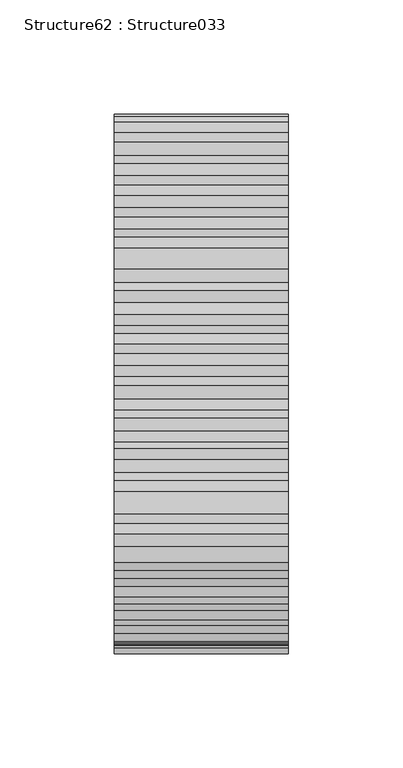
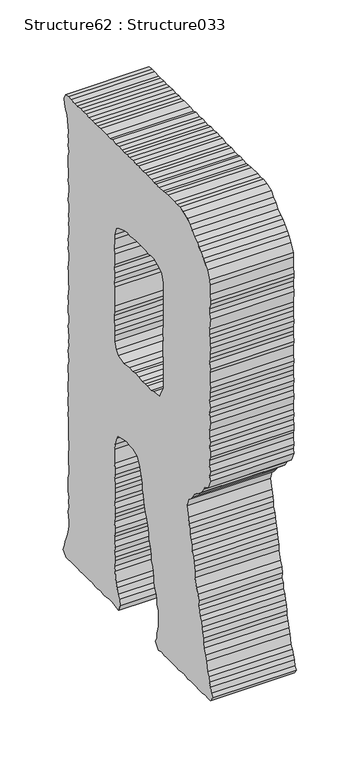
"""IFC4 building model written with IfcOpenShell, lengths in millimetres: proxy geometry, Structure62 : Structure033."""

import ifcopenshell
import ifcopenshell.guid

model = None  # the IFC model being written
_history = None  # IfcOwnerHistory: only IFC2X3 demands one
_inside = {}  # id of a spatial element -> (the spatial element, [elements in it])
_under = {}  # id of a project, library or spatial element -> (it, [spatial elements below it])
_declared = {}  # id of a project -> (the project, [libraries it declares])
_typed = {}  # id of a type object -> (the type object, [elements of that type])
_made_of = {}  # id of a material, layer set ... -> (it, [elements and type objects made of it])


def new_model(schema):
    """Start an empty IFC model of exactly this schema.

    Asked for "IFC4X3", IfcOpenShell would pick the latest addendum, in which some entities
    have other attributes; the version numbers below select the first issue.
    IFC2X3 requires an IfcOwnerHistory on every rooted entity: one is made here for all.
    """
    global model, _history
    if schema == "IFC4X3":
        model = ifcopenshell.file(schema_version=(4, 3, 0, 0))
    else:
        model = ifcopenshell.file(schema=schema)
    _inside.clear()
    _under.clear()
    _declared.clear()
    _typed.clear()
    _made_of.clear()
    _history = None
    if model.schema == "IFC2X3":
        org = make("IfcOrganization", Name="unknown")
        user = make(
            "IfcPersonAndOrganization",
            ThePerson=make("IfcPerson", FamilyName="unknown"),
            TheOrganization=org,
        )
        app = make(
            "IfcApplication",
            ApplicationDeveloper=org,
            Version="unknown",
            ApplicationFullName="unknown",
            ApplicationIdentifier="unknown",
        )
        _history = make(
            "IfcOwnerHistory",
            OwningUser=user,
            OwningApplication=app,
            ChangeAction="ADDED",
            CreationDate=0,
        )
    return model


def make(cls, **values):
    """One entity of the class cls with the attributes given. An attribute that is None is left unset."""
    return model.create_entity(
        cls, **{name: value for name, value in values.items() if value is not None}
    )


def rooted(cls, **values):
    """An entity with a GlobalId (a new one), such as an element, a storey or a relation."""
    return make(cls, GlobalId=ifcopenshell.guid.new(), OwnerHistory=_history, **values)


def si_unit(unit_type, name, prefix=None):
    """IfcSIUnit, for example si_unit("LENGTHUNIT", "METRE", prefix="MILLI")."""
    return make("IfcSIUnit", UnitType=unit_type, Prefix=prefix, Name=name)


def assignment(units):
    """IfcUnitAssignment: the units of a project."""
    return None if units is None else make("IfcUnitAssignment", Units=units)


def point(xyz):
    """IfcCartesianPoint."""
    return None if xyz is None else make("IfcCartesianPoint", Coordinates=xyz)


def direction(xyz):
    """IfcDirection."""
    return None if xyz is None else make("IfcDirection", DirectionRatios=xyz)


def frame(location, z_axis=None, x_axis=None):
    """IfcAxis2Placement3D, a coordinate frame: its origin and axes. An axis left out is left unset."""
    return make(
        "IfcAxis2Placement3D",
        Location=point(location),
        Axis=direction(z_axis),
        RefDirection=direction(x_axis),
    )


def origin():
    """The frame at (0, 0, 0) with its axes left unset."""
    return frame((0.0, 0.0, 0.0))


def place(relative_to, where):
    """IfcLocalPlacement: puts the frame where relative to a parent placement (None: the world)."""
    return make(
        "IfcLocalPlacement", PlacementRelTo=relative_to, RelativePlacement=where
    )


def context(
    kind, dimensions, precision=None, world=None, true_north=None, identifier=None
):
    """IfcGeometricRepresentationContext, for example the 3D "Model" context."""
    return make(
        "IfcGeometricRepresentationContext",
        ContextIdentifier=identifier,
        ContextType=kind,
        CoordinateSpaceDimension=dimensions,
        Precision=precision,
        WorldCoordinateSystem=world,
        TrueNorth=true_north,
    )


def project(units=None, contexts=None):
    """IfcProject with its units and contexts."""
    return rooted(
        "IfcProject",
        Name="project",
        RepresentationContexts=contexts,
        UnitsInContext=assignment(units),
    )


def spatial(cls, under=None, at=None, **own):
    """A site, building, storey or space (cls), placed at a placement, below another one or the project."""
    s = rooted(cls, ObjectPlacement=at, **own)
    if under is not None:
        _under.setdefault(under.id(), (under, []))[1].append(s)
    return s


def polyline(points):
    """IfcPolyline through the points."""
    return make("IfcPolyline", Points=[point(p) for p in points])


def outline(outer, holes=None, kind="AREA"):
    """IfcArbitraryClosedProfileDef: a profile drawn as a closed curve; with holes, ...WithVoids."""
    if holes is None:
        return make("IfcArbitraryClosedProfileDef", ProfileType=kind, OuterCurve=outer)
    return make(
        "IfcArbitraryProfileDefWithVoids",
        ProfileType=kind,
        OuterCurve=outer,
        InnerCurves=holes,
    )


def extrude(swept, where, along, depth):
    """IfcExtrudedAreaSolid: the profile swept, set in the frame where, extruded along a direction by depth."""
    return make(
        "IfcExtrudedAreaSolid",
        SweptArea=swept,
        Position=where,
        ExtrudedDirection=direction(along),
        Depth=depth,
    )


def shape(context_of_items, identifier, shape_type, items):
    """IfcShapeRepresentation: the items that make up one representation, for example the "Body"."""
    return make(
        "IfcShapeRepresentation",
        ContextOfItems=context_of_items,
        RepresentationIdentifier=identifier,
        RepresentationType=shape_type,
        Items=items,
    )


def source(mapping_origin, context_of_items, identifier, shape_type, items):
    """IfcRepresentationMap: a shape defined once, which mapped items show again and again."""
    return make(
        "IfcRepresentationMap",
        MappingOrigin=mapping_origin,
        MappedRepresentation=shape(context_of_items, identifier, shape_type, items),
    )


def transform(
    local_origin,
    x_axis=None,
    y_axis=None,
    z_axis=None,
    scale=None,
    scale2=None,
    scale3=None,
    uniform=True,
):
    """IfcCartesianTransformationOperator3D, or its non-uniform kind. x_axis, y_axis, z_axis: its Axis1, 2, 3."""
    if uniform:
        return make(
            "IfcCartesianTransformationOperator3D",
            Axis1=direction(x_axis),
            Axis2=direction(y_axis),
            LocalOrigin=point(local_origin),
            Scale=scale,
            Axis3=direction(z_axis),
        )
    return make(
        "IfcCartesianTransformationOperator3DnonUniform",
        Axis1=direction(x_axis),
        Axis2=direction(y_axis),
        LocalOrigin=point(local_origin),
        Scale=scale,
        Axis3=direction(z_axis),
        Scale2=scale2,
        Scale3=scale3,
    )


def mapped(mapping_source, mapping_target):
    """IfcMappedItem: shows the shape of a source again, moved by a transform."""
    return make(
        "IfcMappedItem", MappingSource=mapping_source, MappingTarget=mapping_target
    )


def made_of(thing, what):
    """Note that an element or type object is made of a material, layer set ...; save() writes the relation."""
    if what is not None:
        _made_of.setdefault(what.id(), (what, []))[1].append(thing)
    return thing


def element(
    cls,
    number,
    at=None,
    inside=None,
    cuts=None,
    type_object=None,
    material=None,
    context=None,
    identifier="Body",
    shape_type=None,
    held_by="IfcProductDefinitionShape",
    body=None,
    shapes=None,
    **own,
):
    """One element of the class cls, such as IfcWall. Its Tag is "e" and its number.

    at: its placement. inside: the storey or other place that contains it. cuts: it is an
    opening in that element (IfcRelVoidsElement). A single representation is given by context,
    identifier, shape_type and body (its items); several are given by shapes. held_by: the class
    of the entity that holds the representations. save() writes the other relations.
    """
    e = rooted(cls, Tag="e%d" % number, ObjectPlacement=at, **own)
    if body is not None:
        shapes = [shape(context, identifier, shape_type, body)]
    if shapes is not None:
        e.Representation = make(held_by, Representations=shapes)
    if inside is not None:
        _inside.setdefault(inside.id(), (inside, []))[1].append(e)
    if cuts is not None:
        rooted(
            "IfcRelVoidsElement", RelatingBuildingElement=cuts, RelatedOpeningElement=e
        )
    if type_object is not None:
        _typed.setdefault(type_object.id(), (type_object, []))[1].append(e)
    return made_of(e, material)


def aggregate(whole, parts):
    """IfcRelAggregates: a whole, such as a stair, and the parts it consists of."""
    return rooted("IfcRelAggregates", RelatingObject=whole, RelatedObjects=parts)


def save(model, path):
    """Write the relations noted so far, then the file.

    IfcRelAggregates (storeys below a building ...), IfcRelContainedInSpatialStructure (elements
    in a storey), IfcRelDefinesByType, IfcRelAssociatesMaterial and IfcRelDeclares: one each for
    every whole, place, type object, material and project.
    """
    for whole, parts in _under.values():
        aggregate(whole, parts)
    for where, things in _inside.values():
        rooted(
            "IfcRelContainedInSpatialStructure",
            RelatedElements=things,
            RelatingStructure=where,
        )
    for kind, things in _typed.values():
        rooted("IfcRelDefinesByType", RelatedObjects=things, RelatingType=kind)
    for what, things in _made_of.values():
        rooted("IfcRelAssociatesMaterial", RelatedObjects=things, RelatingMaterial=what)
    for by, libraries in _declared.values():
        rooted("IfcRelDeclares", RelatingContext=by, RelatedDefinitions=libraries)
    model.write(path)


def structure62_structure033_9c90971f(model_context):
    return source(origin(), model_context, "Body", "SweptSolid", [
        extrude(outline(polyline([(274499.2360937, 3899.7046941), (274499.8378204, 3903.2059411), (274499.8378204, 3907.888177), (274498.6568315, 3918.4480792), (274499.8378204, 3923.1319197), (274499.8378204, 3927.8077372), (274498.6568315, 3932.4899731), (274498.6568315, 3936.0345445), (274499.2360937, 3941.8753048), (274499.2360937, 3951.2606365), (274499.8378204, 3955.360401), (274503.3358582, 3962.9774586), (274506.8579651, 3967.6789497), (274509.1974785, 3970.5768654), (274513.2988475, 3974.1214368), (274516.2400876, 3977.6194746), (274519.1588632, 3979.9621971), (274523.8619589, 3982.8793681), (274527.3616013, 3987.0048063), (274530.8821036, 3989.9460463), (274534.381746, 3994.0233463), (274541.4227505, 3996.390138), (274546.7051085, 3997.5486624), (274551.3857399, 3996.9645864), (274555.4855043, 3997.5486624), (274565.4484937, 3997.5486624), (274570.1499848, 3996.9645864), (274573.6496272, 3996.390138), (274579.5112475, 3996.390138), (274584.2127386, 3996.9645864), (274587.1331188, 3996.390138), (274591.8121455, 3996.390138), (274597.6737657, 3996.9645864), (274601.1734081, 3996.9645864), (274605.8748993, 3996.390138), (274611.7365195, 3997.5486624), (274615.836284, 3996.9645864), (274620.5393798, 3997.5486624), (274625.7992733, 3996.9645864), (274629.8990378, 3997.5486624), (274634.5796691, 3996.390138), (274638.1001714, 3996.9645864), (274642.8032672, 3997.5486624), (274648.0631607, 3996.390138), (274653.3230543, 3997.5486624), (274656.8435565, 3996.390138), (274662.7051767, 3996.9645864), (274672.0872992, 3996.9645864), (274676.7679305, 3996.390138), (274680.2884328, 3996.9645864), (274685.5707908, 3996.390138), (274689.6705553, 3996.9645864), (274694.9304488, 3996.9645864), (274699.6110801, 3996.390138), (274703.7333091, 3996.9645864), (274708.9932026, 3996.390138), (274712.5137049, 3996.390138), (274718.3753251, 3996.9645864), (274722.4766942, 3996.9645864), (274727.1781854, 3996.390138), (274729.4968389, 3991.6806238), (274728.9175767, 3986.4046842), (274727.1781854, 3981.7208437), (274724.8162076, 3978.2035506), (274723.6576831, 3973.5197101), (274722.4766942, 3963.5615346), (274723.0559564, 3959.4617701), (274722.4766942, 3954.7506513), (274723.0559564, 3949.4923624), (274721.8749675, 3944.8165449), (274723.0559564, 3939.5325823), (274723.0559564, 3930.1745289), (274722.4766942, 3926.6492128), (274722.4766942, 3920.7908018), (274723.0559564, 3916.0909152), (274721.8749675, 3911.4054701), (274721.8749675, 3906.7328618), (274722.4766942, 3903.2059411), (274723.0559564, 3897.3475301), (274721.8749675, 3893.822214), (274721.8749675, 3887.9621984), (274722.4766942, 3883.2863809), (274721.8749675, 3878.5784713), (274722.4766942, 3875.0772243), (274721.8749675, 3870.4030114), (274721.8749675, 3865.7015202), (274723.0559564, 3859.8591552), (274722.4766942, 3855.7353217), (274723.0559564, 3850.4754282), (274721.8749675, 3846.3772683), (274721.8749675, 3841.0900965), (274722.4766942, 3836.9919366), (274723.0559564, 3831.732043), (274722.4766942, 3828.2163546), (274722.4766942, 3818.2309008), (274721.8749675, 3812.9726119), (274722.4766942, 3809.4729695), (274723.0559564, 3803.5872802), (274722.4766942, 3798.9050443), (274723.0559564, 3794.8309535), (274723.0559564, 3789.5293402), (274721.8749675, 3786.0280932), (274721.8749675, 3780.1616592), (274723.0559564, 3776.6427615), (274722.4766942, 3771.9605256), (274721.8749675, 3766.1021146), (274722.4766942, 3761.418274), (274721.8749675, 3757.8753073), (274723.0559564, 3752.6170184), (274722.4766942, 3747.9428055), (274721.8749675, 3742.6748889), (274723.0559564, 3738.5574738), (274723.0559564, 3733.2991849), (274722.4766942, 3729.1737467), (274722.4766942, 3725.0996559), (274723.0559564, 3720.4158154), (274723.0559564, 3714.5301261), (274722.4766942, 3709.8559132), (274723.0559564, 3706.3289925), (274723.0559564, 3701.6547796), (274722.4766942, 3695.786741), (274723.0559564, 3691.0868544), (274722.4766942, 3686.4030139), (274722.4766942, 3668.2437048), (274721.8749675, 3663.5598643), (274721.8749675, 3658.8840468), (274722.4766942, 3654.1841602), (274722.4766942, 3645.4262289), (274721.8749675, 3639.5405396), (274721.8749675, 3634.856699), (274723.0559564, 3630.1824862), (274723.0559564, 3616.69739), (274721.8749675, 3612.0135494), (274722.4766942, 3607.8961343), (274721.8749675, 3602.0280957), (274723.0559564, 3597.9540049), (274721.8749675, 3588.5702778), (274721.8749675, 3583.8864372), (274724.2369453, 3574.5107332), (274725.4179342, 3570.9854171), (274727.7574476, 3565.7094775), (274728.9175767, 3561.6257591), (274730.6778278, 3556.3417965), (274726.5764587, 3551.0658569), (274722.4766942, 3551.0658569), (274718.3753251, 3551.6675836), (274708.4139404, 3551.6675836), (274704.3125713, 3551.0658569), (274699.6110801, 3551.6675836), (274689.6705553, 3551.6675836), (274684.9690641, 3552.242032), (274680.8901595, 3551.0658569), (274676.1886683, 3551.0658569), (274672.0872992, 3551.6675836), (274667.4066679, 3551.0658569), (274662.1259145, 3551.6675836), (274658.0245454, 3552.242032), (274653.9247809, 3552.242032), (274649.2441496, 3551.0658569), (274643.3825294, 3550.4833855), (274641.0205516, 3556.3417965), (274642.2015405, 3561.6257591), (274644.5635183, 3565.1254015), (274645.7011829, 3570.9854171), (274647.4838985, 3574.5107332), (274648.6424229, 3585.0706354), (274649.8234119, 3589.1527492), (274649.2441496, 3594.4286888), (274649.2441496, 3597.9540049), (274649.8234119, 3602.6298224), (274648.6424229, 3607.8961343), (274649.8234119, 3613.1720739), (274649.8234119, 3617.2718384), (274648.6424229, 3621.3732075), (274648.6424229, 3626.0554434), (274649.8234119, 3631.915459), (274649.2441496, 3636.6153456), (274648.6424229, 3640.114988), (274648.6424229, 3644.8245022), (274649.8234119, 3650.1004418), (274649.2441496, 3654.1841602), (274649.2441496, 3660.0682449), (274648.6424229, 3664.7440624), (274649.2441496, 3668.2437048), (274649.8234119, 3672.9435914), (274648.6424229, 3677.6274319), (274648.6424229, 3683.4858429), (274649.8234119, 3688.1873341), (274649.8234119, 3701.6547796), (274648.6424229, 3706.9130685), (274646.8821718, 3713.9556777), (274643.9617916, 3717.4729707), (274635.7606581, 3719.8140887), (274629.8990378, 3720.9726131), (274626.3785356, 3719.8140887), (274620.5393798, 3719.8140887), (274613.4967707, 3716.8985223), (274609.3970062, 3709.2718371), (274608.2144127, 3703.4134261), (274606.476626, 3698.711935), (274605.2956371, 3695.2122926), (274605.2956371, 3689.3458585), (274604.1146482, 3685.2444894), (274602.9336593, 3679.9701544), (274602.3543971, 3675.8687854), (274600.5925413, 3670.5848228), (274599.4340169, 3667.0851803), (274597.6737657, 3662.3836892), (274596.4927768, 3657.7014533), (274595.3342524, 3652.4431643), (274595.3342524, 3648.3161216), (274594.1532635, 3644.2420307), (274592.4138722, 3639.5405396), (274591.8121455, 3634.856699), (274591.2328833, 3629.5984101), (274588.8933699, 3625.472972), (274588.2916433, 3620.7971545), (274587.712381, 3616.0972679), (274587.1331188, 3611.4134274), (274585.9505253, 3606.1551384), (274583.6110119, 3602.0280957), (274583.0317497, 3596.7698067), (274582.4524875, 3592.6700423), (274580.0905097, 3588.5702778), (274580.0905097, 3583.2863152), (274580.0905097, 3573.9266571), (274581.2714986, 3570.4109687), (274582.4524875, 3565.1254015), (274583.0317497, 3560.441561), (274584.7920009, 3556.3417965), (274580.0905097, 3550.4833855), (274575.4098784, 3551.6675836), (274571.3085093, 3550.4833855), (274567.2087448, 3551.0658569), (274553.7252532, 3551.0658569), (274547.863633, 3550.4833855), (274543.1846063, 3551.6675836), (274539.6849639, 3551.6675836), (274533.8008792, 3550.4833855), (274529.7011147, 3551.6675836), (274520.9207189, 3551.6675836), (274516.2400876, 3551.0658569), (274510.9577296, 3551.0658569), (274506.2787029, 3551.6675836), (274502.756596, 3551.0658569), (274498.0551048, 3551.6675836), (274494.5554624, 3556.3417965), (274496.8949758, 3559.2669905), (274498.0551048, 3564.54293), (274499.8378204, 3568.0682461), (274500.9963449, 3572.7440636), (274503.3358582, 3576.2693797), (274505.097714, 3585.0706354), (274506.2787029, 3590.3289243), (274508.6182162, 3595.5872132), (274509.7992051, 3600.2967274), (274509.7992051, 3604.3964919), (274510.9577296, 3609.6547808), (274512.1178586, 3613.772196), (274512.7195853, 3619.0385079), (274515.0590987, 3622.555801), (274515.6383609, 3627.8397636), (274517.4210765, 3631.3410106), (274516.8193498, 3636.6153456), (274517.9778743, 3641.8832621), (274520.3189922, 3646.557475), (274522.68097, 3654.7842823), (274522.68097, 3660.6250426), (274523.8619589, 3665.3265338), (274524.4412212, 3670.0007467), (274525.5997456, 3674.1277895), (274527.3616013, 3678.2018803), (274527.9408636, 3683.4858429), (274529.1218525, 3687.587212), (274530.8821036, 3691.6869765), (274530.8821036, 3696.9709391), (274532.0630925, 3701.0723082), (274533.221617, 3706.9130685), (274535.5627349, 3716.2887726), (274533.221617, 3723.9154578), (274530.3028414, 3726.2742264), (274527.3616013, 3729.7738688), (274523.8619589, 3734.47536), (274519.73973, 3737.9750024), (274516.8193498, 3739.7416719), (274512.7195853, 3743.2332913), (274509.7992051, 3747.9428055), (274506.8579651, 3751.4424479), (274502.756596, 3753.8012165), (274498.6568315, 3762.5848215), (274499.8378204, 3766.684586), (274498.6568315, 3771.3860772), (274499.8378204, 3777.2444882), (274499.8378204, 3781.9299333), (274498.6568315, 3785.4456218), (274498.6568315, 3790.7039107), (274499.8378204, 3794.8309535), (274498.6568315, 3800.0876378), (274499.8378204, 3804.1890069), (274499.8378204, 3810.0474179), (274498.6568315, 3818.2309008), (274499.2360937, 3823.5341187), (274499.8378204, 3827.6162325), (274498.6568315, 3832.8921721), (274499.8378204, 3838.1761347), (274499.2360937, 3842.8583706), (274499.2360937, 3846.9757858), (274498.6568315, 3851.6612309), (274499.2360937, 3856.9179152), (274499.2360937, 3866.8776953), (274498.6568315, 3870.4030114), (274499.8378204, 3876.263027), (274499.2360937, 3880.3627915), (274499.2360937, 3884.4609514), (274498.6568315, 3890.320967), (274499.2360937, 3894.4030808), (274499.2360937, 3899.7046941)]), holes=[polyline([(274626.3785356, 3794.8309535), (274634.5796691, 3793.6451507), (274643.3825294, 3795.960595), (274646.3029096, 3800.0876378), (274649.2441496, 3805.9476534), (274648.6424229, 3811.7884138), (274648.6424229, 3816.4883003), (274649.2441496, 3820.5896694), (274649.8234119, 3825.849563), (274649.8234119, 3830.5574726), (274648.6424229, 3834.6588416), (274649.2441496, 3839.9331766), (274649.2441496, 3858.1021133), (274649.8234119, 3861.6178018), (274648.6424229, 3867.4601667), (274649.2441496, 3871.5599312), (274649.8234119, 3876.8438938), (274648.6424229, 3880.3627915), (274648.6424229, 3890.320967), (274649.8234119, 3894.4030808), (274648.6424229, 3904.9645876), (274648.6424229, 3909.0627475), (274646.3029096, 3916.0909152), (274642.8032672, 3918.4480792), (274634.5796691, 3921.3748778), (274629.8990378, 3922.5494483), (274625.2200111, 3921.3748778), (274621.6979043, 3921.9733953), (274615.836284, 3922.5494483), (274601.1734081, 3922.5494483), (274596.4927768, 3921.3748778), (274592.97067, 3922.5494483), (274588.2916433, 3922.5494483), (274579.5112475, 3919.0321552), (274576.011605, 3915.5068392), (274573.070365, 3908.46423), (274573.6496272, 3904.3901392), (274573.070365, 3900.2887701), (274573.070365, 3895.0048075), (274573.6496272, 3890.905043), (274573.070365, 3885.6210804), (274573.6496272, 3880.9452629), (274573.6496272, 3876.8438938), (274573.070365, 3871.5599312), (274573.070365, 3867.4601667), (274574.2288895, 3862.2018778), (274574.2288895, 3858.1021133), (274573.6496272, 3854.0007442), (274574.2288895, 3849.3008577), (274574.2288895, 3839.9331766), (274573.6496272, 3834.0474873), (274573.6496272, 3829.374879), (274573.070365, 3825.2911606), (274573.070365, 3820.015221), (274573.6496272, 3816.4883003), (274573.6496272, 3810.6298893), (274573.070365, 3806.5317294), (274577.1701295, 3800.0876378), (274578.9095208, 3795.960595), (274587.712381, 3794.8309535), (274591.8121455, 3793.6451507), (274597.6737657, 3794.2292268), (274601.1734081, 3794.2292268), (274605.8748993, 3793.6451507), (274611.1572573, 3794.8309535), (274616.9964131, 3794.8309535), (274620.5393798, 3794.2292268), (274626.3785356, 3794.8309535)])]), frame((-59031.6926606, 0.0, 0.0), z_axis=(1.0, 0.0, 0.0), x_axis=(0.0, 1.0, 0.0)), (0.0, 0.0, 1.0), 76.2),
    ])


if __name__ == "__main__":
    model = new_model("IFC4")
    model_context = context("Model", 3, world=origin())
    ifc_project = project(units=[si_unit("LENGTHUNIT", "METRE", prefix="MILLI")], contexts=[model_context])
    site = spatial("IfcSite", under=ifc_project)
    building = spatial("IfcBuilding", under=site)
    placement = place(None, origin())
    structure62_structure033_shape = structure62_structure033_9c90971f(model_context)
    element("IfcBuildingElementProxy", 1, Name="Structure62 : Structure033", ObjectType="Structure62 : Structure033", at=placement, inside=building, context=model_context, shape_type="MappedRepresentation", body=[
        mapped(structure62_structure033_shape, transform((0.0, 0.0, 0.0), x_axis=(1.0, 0.0, 0.0), y_axis=(0.0, 1.0, 0.0), z_axis=(0.0, 0.0, 1.0))),
    ])
    save(model, "model.ifc")

# Revit data of these elements
# Type "Structure62 : Structure033"
#   NameOverride = "Structure033"
# Element 1 (IfcBuildingElementProxy, "Structure62 : Structure033")
#   Materials on its faces: "BRUSHED ALUM. LETTERING"
# Materials
#   "BRUSHED ALUM. LETTERING": class "Unassigned", colour RGB 169 181 186, transparency 0, Cost = 0
